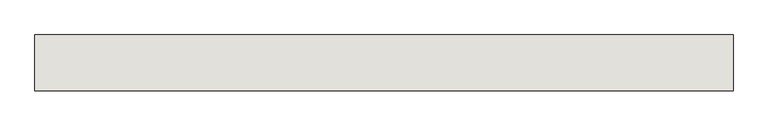
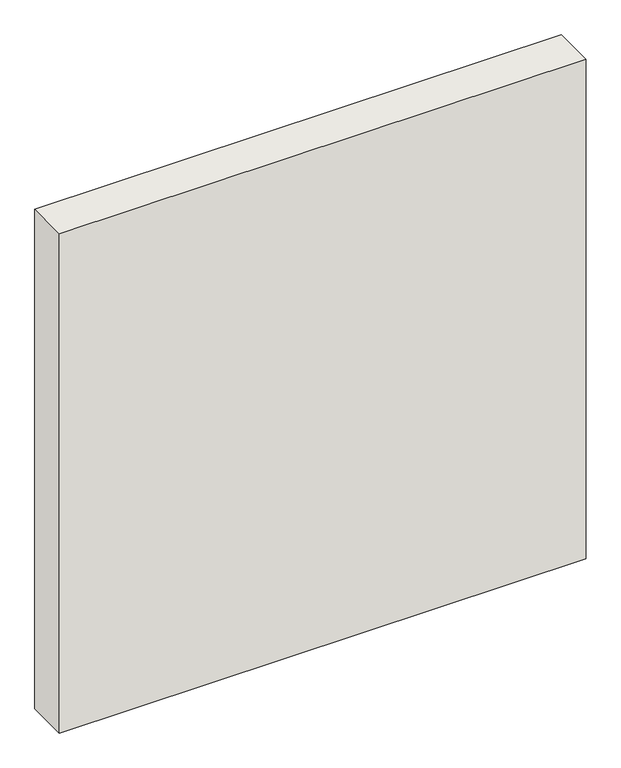
"""IFC4 building model written with IfcOpenShell, lengths in millimetres: wall geometry, Holzwand."""

from ifc_helpers import new_model, si_unit, origin, origin_with_axes, place, context, project, spatial, polyline, outline, extrude, source, transform, mapped, element, save


def wall_f22dd5b5(model_context):
    return source(origin(), model_context, "Body", "SweptSolid", [
        extrude(outline(polyline([(0.0, 200.0), (2495.0, 200.0), (2495.0, 0.0), (0.0, 0.0), (0.0, 200.0)])), origin_with_axes(), (0.0, 0.0, 1.0), 2500.0),
    ])


if __name__ == "__main__":
    model = new_model("IFC4")
    model_context = context("Model", 3, world=origin())
    ifc_project = project(units=[si_unit("LENGTHUNIT", "METRE", prefix="MILLI")], contexts=[model_context])
    site = spatial("IfcSite", under=ifc_project)
    building = spatial("IfcBuilding", under=site)
    placement = place(None, origin())
    wall_shape = wall_f22dd5b5(model_context)
    element("IfcWall", 1, ObjectType="Holzwand", at=placement, inside=building, context=model_context, shape_type="MappedRepresentation", body=[
        mapped(wall_shape, transform((0.0, 0.0, 0.0), x_axis=(1.0, 0.0, 0.0), y_axis=(0.0, 1.0, 0.0), z_axis=(0.0, 0.0, 1.0))),
    ])
    save(model, "model.ifc")

# Revit data of these elements
# Element 1 (IfcWall, "Holzwand")
#   Materials on its faces: "holzschalung"
# Materials
#   "holzschalung": class "Unassigned", colour RGB 128 128 128, transparency 0
